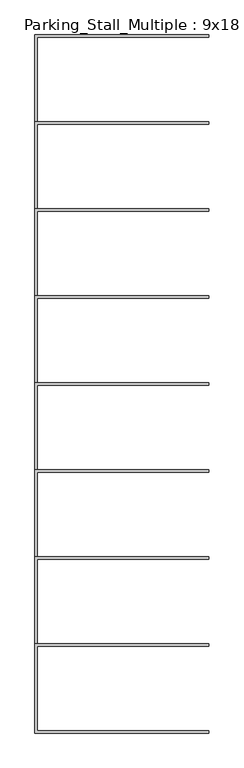
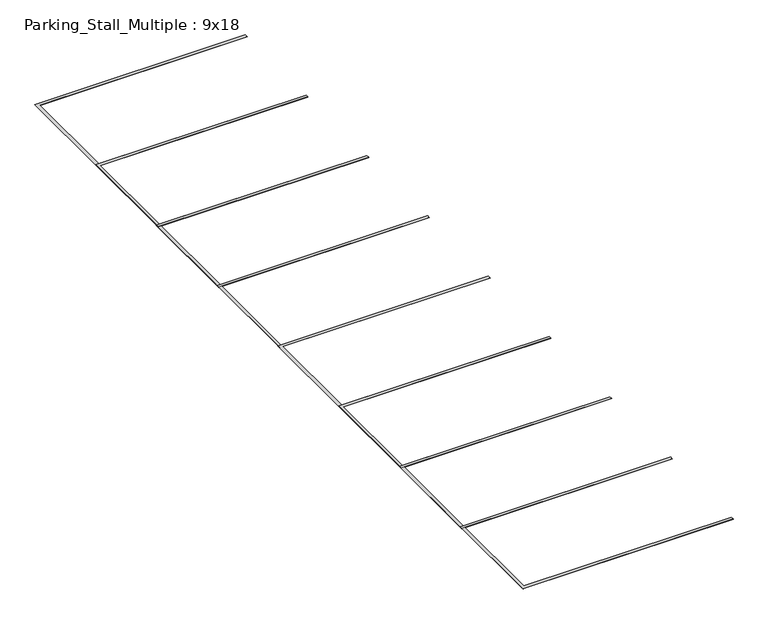
"""IFC4 building model written with IfcOpenShell, lengths in millimetres: proxy geometry, Parking_Stall_Multiple : 9x18."""

from ifc_helpers import new_model, si_unit, origin, origin_with_axes, place, context, project, spatial, polyline, outline, extrude, source, transform, mapped, element, save


def parking_stall_multiple_9x18_69ab94fe(model_context):
    return source(origin(), model_context, "Body", "SweptSolid", [
        extrude(outline(polyline([(5486.4, -19202.4), (5486.4, -19278.6), (76.2, -19278.6), (76.2, -21945.6), (5486.4, -21945.6), (5486.4, -22021.8), (0.0, -22021.8), (0.0, -19202.4), (5486.4, -19202.4)])), origin_with_axes(), (0.0, 0.0, 1.0), 6.35),
        extrude(outline(polyline([(5486.4, -16459.2), (5486.4, -16535.4), (76.2, -16535.4), (76.2, -19202.4), (5486.4, -19202.4), (5486.4, -19278.6), (0.0, -19278.6), (0.0, -16459.2), (5486.4, -16459.2)])), origin_with_axes(), (0.0, 0.0, 1.0), 6.35),
        extrude(outline(polyline([(5486.4, -13716.0), (5486.4, -13792.2), (76.2, -13792.2), (76.2, -16459.2), (5486.4, -16459.2), (5486.4, -16535.4), (0.0, -16535.4), (0.0, -13716.0), (5486.4, -13716.0)])), origin_with_axes(), (0.0, 0.0, 1.0), 6.35),
        extrude(outline(polyline([(5486.4, -10972.8), (5486.4, -11049.0), (76.2, -11049.0), (76.2, -13716.0), (5486.4, -13716.0), (5486.4, -13792.2), (0.0, -13792.2), (0.0, -10972.8), (5486.4, -10972.8)])), origin_with_axes(), (0.0, 0.0, 1.0), 6.35),
        extrude(outline(polyline([(5486.4, -8229.6), (5486.4, -8305.8), (76.2, -8305.8), (76.2, -10972.8), (5486.4, -10972.8), (5486.4, -11049.0), (0.0, -11049.0), (0.0, -8229.6), (5486.4, -8229.6)])), origin_with_axes(), (0.0, 0.0, 1.0), 6.35),
        extrude(outline(polyline([(5486.4, -5486.4), (5486.4, -5562.6), (76.2, -5562.6), (76.2, -8229.6), (5486.4, -8229.6), (5486.4, -8305.8), (0.0, -8305.8), (0.0, -5486.4), (5486.4, -5486.4)])), origin_with_axes(), (0.0, 0.0, 1.0), 6.35),
        extrude(outline(polyline([(5486.4, -2743.2), (5486.4, -2819.4), (76.2, -2819.4), (76.2, -5486.4), (5486.4, -5486.4), (5486.4, -5562.6), (0.0, -5562.6), (0.0, -2743.2), (5486.4, -2743.2)])), origin_with_axes(), (0.0, 0.0, 1.0), 6.35),
        extrude(outline(polyline([(5486.4, 0.0), (5486.4, -76.2), (76.2, -76.2), (76.2, -2743.2), (5486.4, -2743.2), (5486.4, -2819.4), (0.0, -2819.4), (0.0, 0.0), (5486.4, 0.0)])), origin_with_axes(), (0.0, 0.0, 1.0), 6.35),
    ])


if __name__ == "__main__":
    model = new_model("IFC4")
    model_context = context("Model", 3, world=origin())
    ifc_project = project(units=[si_unit("LENGTHUNIT", "METRE", prefix="MILLI")], contexts=[model_context])
    site = spatial("IfcSite", under=ifc_project)
    building = spatial("IfcBuilding", under=site)
    placement = place(None, origin())
    parking_stall_multiple_9x18_shape = parking_stall_multiple_9x18_69ab94fe(model_context)
    element("IfcBuildingElementProxy", 1, Name="Parking_Stall_Multiple : 9x18", ObjectType="Parking_Stall_Multiple : 9x18", at=placement, inside=building, context=model_context, shape_type="MappedRepresentation", body=[
        mapped(parking_stall_multiple_9x18_shape, transform((0.0, 0.0, 0.0), x_axis=(1.0, 0.0, 0.0), y_axis=(0.0, 1.0, 0.0), z_axis=(0.0, 0.0, 1.0))),
    ])
    save(model, "model.ifc")

# Revit data of these elements
# Type "Parking_Stall_Multiple : 9x18"
#   Parking_Width_M = 9' - 0"
#   Parking_Run_Length [instance default] = 65' - 0"
#   Parking_Line_Width = 0' - 3"
#   Parking_Length_M = 18' - 0"
#   Single_Parking_Visibility [instance default] = no
#   Parking_ADA_Symbol = no
#   ParkingUnitsArray [instance default] = 7
#   ParkingUnits [instance default] = 7
#   Multiple_Parking_Visibility [instance default] = yes
#   Parking_Line_Material = none
# Element 1 (IfcBuildingElementProxy, "Parking_Stall_Multiple : 9x18")
#   Parking_Run_Length = 72' - 6.1556"
#   ParkingUnitsArray = 8
#   ParkingUnits = 8
